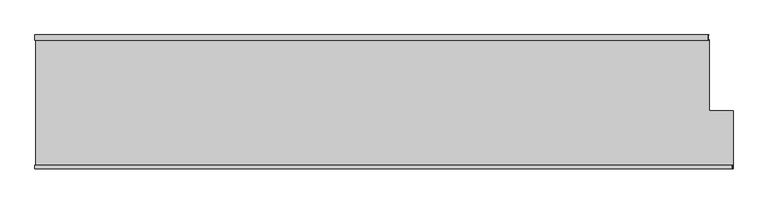
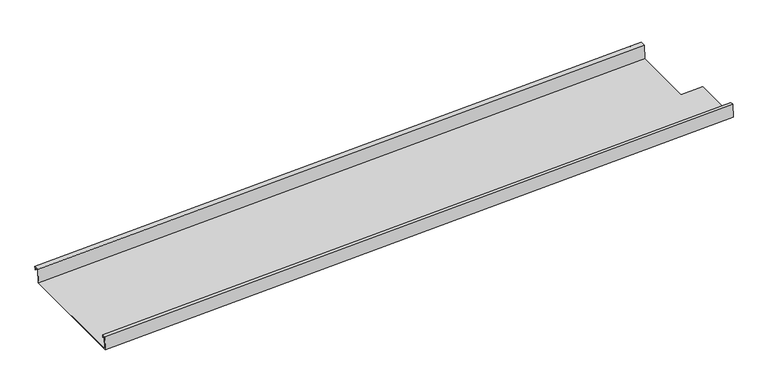
"""IFC4 building model written with IfcOpenShell, lengths in millimetres: proxy geometry, Generic Models 2:Generic Models 2:310765:Generic Models 2:310765 : Generic Models 2:Generic Models 2:310765:81 : Generic Models 2:Generic Models 2:310765:Generic Models 2:310765 : Generic Models 2:Generic Models 2:310765:300385."""

from ifc_helpers import new_model, si_unit, origin, place, context, project, spatial, faceted_brep, source, transform, mapped, element, save


def generic_models_1d5c1cae(model_context):
    return source(origin(), model_context, "Body", "Brep", [
        faceted_brep([(558205.3611715, -578115.660134, 3910.7299065), (558207.4760032, -578115.660134, 3859.9739464), (558207.4760032, -578522.060134, 3859.9739464), (558205.42726, -578522.060134, 3909.1437828), (558205.42726, -578510.947634, 3909.1437828), (558205.823791, -578510.947634, 3899.6270403), (558205.823791, -578512.535134, 3899.6270403), (558205.4933485, -578512.535134, 3907.557659), (558205.4933485, -578520.472634, 3907.557659), (558207.4099147, -578520.472634, 3861.5600702), (558207.4099147, -578117.247634, 3861.5600702), (558205.2950831, -578117.247634, 3912.3160303), (558205.2950831, -578099.785134, 3912.3160303), (558205.7577025, -578099.785134, 3901.213164), (558205.7577025, -578101.372634, 3901.213164), (558205.3611715, -578101.372634, 3910.7299065), (560404.1496034, -578520.472634, 3953.0908905), (560402.2330372, -578520.472634, 3999.0884794), (560402.2330372, -578512.535134, 3999.0884794), (560402.5634797, -578512.535134, 3991.1578606), (560402.5634797, -578510.947634, 3991.1578606), (560402.1669487, -578510.947634, 4000.6746031), (560402.1669487, -578522.060134, 4000.6746031), (560404.2156919, -578522.060134, 3951.5047668), (560404.2156919, -578337.910134, 3951.5047668), (560404.1496034, -578337.910134, 3953.0908905), (560326.4711757, -578101.372634, 3999.10949), (560326.4711757, -578115.660134, 3999.10949), (560326.8677066, -578101.372634, 3989.5927475), (560326.8677066, -578099.785134, 3989.5927475), (560326.4050872, -578099.785134, 4000.6956138), (560326.4050872, -578117.247634, 4000.6956138), (560328.5199189, -578117.247634, 3949.9396537), (560328.5199189, -578337.910134, 3949.9396537), (560328.5199189, -578336.322634, 3949.9396537), (560328.5860074, -578115.660134, 3948.3535299), (560328.5860074, -578337.910134, 3948.3535299)], [[[0, 1, 2, 3, 4, 5, 6, 7, 8, 9, 10, 11, 12, 13, 14, 15]], [[16, 17, 18, 19, 20, 21, 22, 23, 24, 25]], [[0, 15, 26, 27]], [[15, 14, 28, 26]], [[14, 13, 29, 28]], [[13, 12, 30, 29]], [[12, 11, 31, 30]], [[11, 10, 32, 31]], [[10, 9, 16, 25, 33, 34, 32]], [[17, 16, 9, 8]], [[18, 17, 8, 7]], [[19, 18, 7, 6]], [[20, 19, 6, 5]], [[21, 20, 5, 4]], [[22, 21, 4, 3]], [[23, 22, 3, 2]], [[2, 1, 35, 36, 24, 23]], [[1, 0, 27, 35]], [[33, 36, 35, 27, 26, 28, 29, 30, 31, 32, 34]], [[36, 33, 25, 24]]]),
    ])


if __name__ == "__main__":
    model = new_model("IFC4")
    model_context = context("Model", 3, world=origin())
    ifc_project = project(units=[si_unit("LENGTHUNIT", "METRE", prefix="MILLI")], contexts=[model_context])
    site = spatial("IfcSite", under=ifc_project)
    building = spatial("IfcBuilding", under=site)
    placement = place(None, origin())
    generic_models_shape = generic_models_1d5c1cae(model_context)
    element("IfcBuildingElementProxy", 1, Name="Generic Models 2:Generic Models 2:310765:Generic Models 2:310765 : Generic Models 2:Generic Models 2:310765:81 : Generic Models 2:Generic Models 2:310765:Generic Models 2:310765 : Generic Models 2:Generic Models 2:310765:300385", ObjectType="Generic Models 2:Generic Models 2:310765:Generic Models 2:310765 : Generic Models 2:Generic Models 2:310765:81 : Generic Models 2:Generic Models 2:310765:Generic Models 2:310765 : Generic Models 2:Generic Models 2:310765:300385", at=placement, inside=building, context=model_context, shape_type="MappedRepresentation", body=[
        mapped(generic_models_shape, transform((0.0, 0.0, 0.0), x_axis=(1.0, 0.0, 0.0), y_axis=(0.0, 1.0, 0.0), z_axis=(0.0, 0.0, 1.0))),
    ])
    save(model, "model.ifc")

# Revit data of these elements
# Type "Generic Models 2:Generic Models 2:310765:Generic Models 2:310765 : Generic Models 2:Generic Models 2:310765:81 : Generic Models 2:Generic Models 2:310765:Generic Models 2:310765 : Generic Models 2:Generic Models 2:310765:300385"
#   NameOverride = "Generic Models 2:Generic Models 2:310765:Generic Models 2:310765 : Generic Models 2:Generic Models 2:310765:300385"
#   ObjectTypeOverride = "Generic Models 2:310765 : Generic Models 2:Generic Models 2:310765"
#   Reference = "Generic Models 2"
#   Tag = "300385"
# Element 1 (IfcBuildingElementProxy, "Generic Models 2:Generic Models 2:310765:Generic Models 2:310765 : Generic Models 2:Generic Models 2:310765:81 : Generic Models 2:Generic Models 2:310765:Generic Models 2:310765 : Generic Models 2:Generic Models 2:310765:300385")
#   Materials on its faces: "STRUCTURAL STANDING SEAM SHEET METAL ROOFING - BATTENLOK - COLOR T.B.D."
# Materials
#   "STRUCTURAL STANDING SEAM SHEET METAL ROOFING - BATTENLOK - COLOR T.B.D.": class "Generic", colour RGB 120 120 120, transparency 0, Cost = 0
